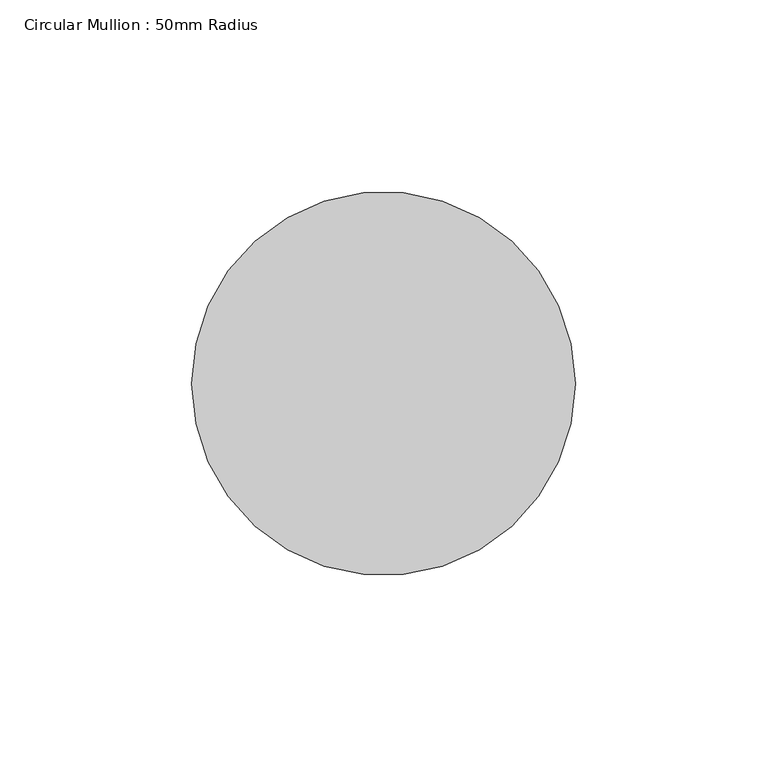
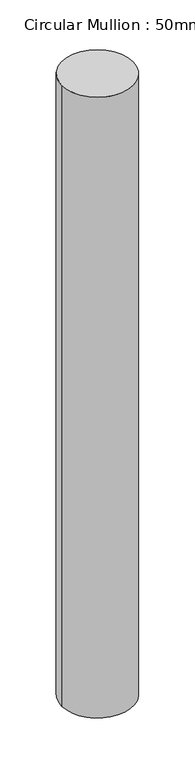
"""IFC4 building model written with IfcOpenShell, lengths in millimetres: member geometry, Circular Mullion : 50mm Radius."""

from ifc_helpers import new_model, si_unit, point, frame, origin, origin_2d, place, context, project, spatial, circle_curve, trimmed, segment, composite_curve, outline, extrude, source, transform, mapped, element, save


def circular_mullion_50mm_radius_30ee8014(model_context):
    return source(origin(), model_context, "Body", "SweptSolid", [
        extrude(outline(composite_curve([segment(trimmed(circle_curve(origin_2d(), 50.0), [point((50.0, 0.0))], [point((-50.0, 0.0))], False, "CARTESIAN"), True, "CONTINUOUS"), segment(trimmed(circle_curve(origin_2d(), 50.0), [point((-50.0, 0.0))], [point((50.0, 0.0))], False, "CARTESIAN"), True, "CONTINUOUS")], self_intersect=False)), frame((0.0, 0.0, -917.979106), z_axis=(0.0, 0.0, 1.0), x_axis=(1.0, 0.0, 0.0)), (0.0, 0.0, 1.0), 917.979106),
    ])


if __name__ == "__main__":
    model = new_model("IFC4")
    model_context = context("Model", 3, world=origin())
    ifc_project = project(units=[si_unit("LENGTHUNIT", "METRE", prefix="MILLI")], contexts=[model_context])
    site = spatial("IfcSite", under=ifc_project)
    building = spatial("IfcBuilding", under=site)
    placement = place(None, origin())
    circular_mullion_50mm_radius_shape = circular_mullion_50mm_radius_30ee8014(model_context)
    element("IfcMember", 1, ObjectType="Circular Mullion : 50mm Radius", at=placement, inside=building, context=model_context, shape_type="MappedRepresentation", body=[
        mapped(circular_mullion_50mm_radius_shape, transform((0.0, 0.0, 0.0), x_axis=(1.0, 0.0, 0.0), y_axis=(0.0, 1.0, 0.0), z_axis=(0.0, 0.0, 1.0))),
    ])
    save(model, "model.ifc")

# Revit data of these elements
# Type "Circular Mullion : 50mm Radius"
#   built-in parameter 1007350 = 0.164042 (stored number, unit not read)
# Element 1 (IfcMember, "Circular Mullion : 50mm Radius")
#   Materials on its faces: "Aluminium"
# Materials
#   "Aluminium": class "Metal", colour RGB 247 247 247, transparency 0, Description = "Aluminium 6061", Cost = 0
